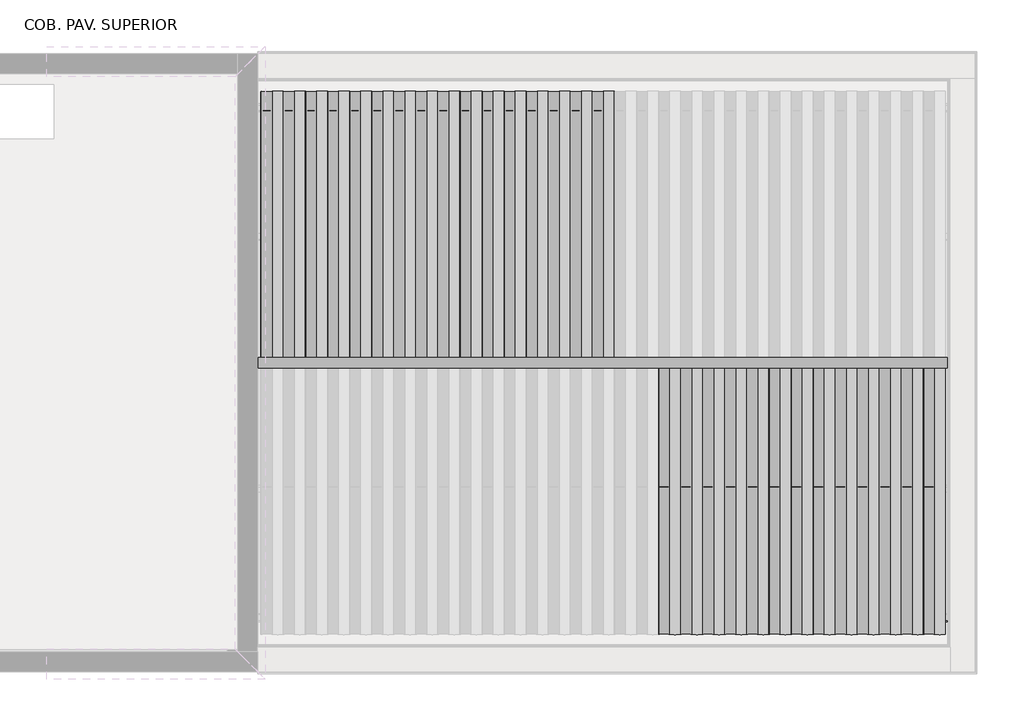
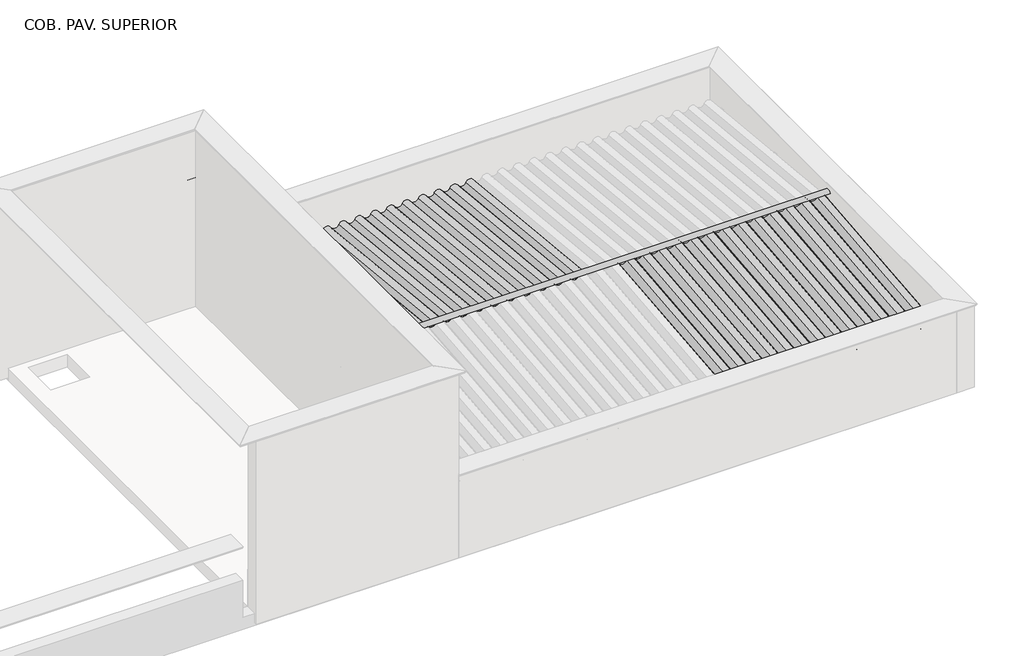
# One storey, part 6 of 7: 39 beams, 8 columns.
# Revit data of these elements (continued)
# Type "Madeira de lei : Berço 6x12cm"
#   A = 0.02 m²
#   Length [instance default] = 1.524 m
#   b = 0.06 m
#   d = 0.12 m
#   Structural Material [instance default] = none
#   Assembly Code = ""
# Type "Cumeeira Telha Ondulada : Fibrocimento"
#   Cost = 5
#   Length [instance default] = 1.524 m
#   b = 0.07 m
#   h = 0.16 m
#   Structural Material = .TELHA DE FIBROCIMENTO
#   Assembly Code = ""
# Type "Telha Ondulada : Fibrocimento"
#   Description = "TELHA ONDULADA FIBROCIMENTO"
#   Cost = 5
#   Length [instance default] = 1.524 m
#   b = 0.07 m
#   h = 0.16 m
#   Structural Material = .TELHA DE FIBROCIMENTO
#   Assembly Code = ""
# Type "Madeira de lei : Viga Cumeeira 6x16cm"
#   A = 0.02 m²
#   Length [instance default] = 1.524 m
#   b = 0.06 m
#   d = 0.16 m
#   Structural Material [instance default] = none
#   Assembly Code = ""
# Type "Madeira de lei-Coluna : Pontalete 6X16cm"
#   A = 0.01952 m²
#   b = 0.06 m
#   d = 0.16 m
#   Structural Material [instance default] = none
#   Assembly Code = ""
# Type "TQS - Pilar retangular : 19.0 x 30.0"
#   b = 0.19 m
#   h = 0.30 m
#   Structural Material [instance default] = Concrete - Cast-in-Place Concrete
# Elements 1, 2, 3, 4, 5, 6, 7, 8 (IfcBeam, "Madeira de lei : Berço 6x12cm")
#   Comments = ""
#   Structural Material = .MADEIRAMENTO
#   Phase Created = CC_PE
#   Materials on its faces: ".MADEIRAMENTO"
# Element 9 (IfcBeam, "Cumeeira Telha Ondulada : Fibrocimento")
#   Comments = ""
#   Phase Created = CC_PE
#   Materials on its faces: ".TELHA DE FIBROCIMENTO"
# Elements 10, 11, 12, 13, 14, 15, 16, 17, 18, 19, 20, 21, 22, 23, 24, 25, 26, 27, 28, 29, 30, 31, 32, 33, 34, 35, 36, 37, 38 (IfcBeam, "Telha Ondulada : Fibrocimento")
#   Phase Created = CC_PE
#   Materials on its faces: ".TELHA DE FIBROCIMENTO"
# Element 39 (IfcBeam, "Madeira de lei : Viga Cumeeira 6x16cm")
#   Comments = ""
#   Structural Material = .MADEIRAMENTO
#   Phase Created = CC_PE
#   Materials on its faces: ".MADEIRAMENTO"
# Elements 40, 41, 42, 43, 44, 45, 46 (IfcColumn, "Madeira de lei-Coluna : Pontalete 6X16cm")
#   Comments = ""
#   Structural Material = .MADEIRAMENTO
#   Phase Created = CC_PE
#   Materials on its faces: ".MADEIRAMENTO"
# Element 47 (IfcColumn, "TQS - Pilar retangular : 19.0 x 30.0")
#   Uso = "ESTRUTURA"
#   Titulo = "PT1"
#   Chave = "PT1//0"
#   Tipo Elemento = "Pilar"
#   SHA1 = "921092CA98E51B071105A8209417B462C0AB35B3"
#   Revisão = ""
#   Tipo de carga = ""
#   Divisor de flexao = ""
#   Secao = "R 19/30 90°"
#   Configuracao = ""
#   Angulo (graus) = ""
#   Detalhamento = ""
#   Casos de vento manual = ""
#   Tipo = ""
#   Alcas = ""
#   Furos = ""
#   Pino = ""
#   Distribuicao = ""
#   Solidarizado = ""
#   Solidarizar na montagem = ""
#   Unir com o próximo = ""
#   Grupo pre moldado = ""
#   Verificado = ""
#   Concreto C = ""
#   Taxa de armadura (kgf/m³) = 0
#   Carga (tf/m²) = 0
#   Carga (tf/m) = 0
#   Carga (tf) = 0
#   Altura = 2.10 m
#   Rebaixo = 0.00 m
#   Altura da fundacao = 0.00 m
#   Largura = 0.00 m
#   Distancia a face = 0.00 m
#   Distancia ao eixo = 0.00 m
#   Resultado de Ensaios fck (MPa) = 0
#   Unique TQS ID = -427
#   Principal = yes
#   Nasce = yes
#   Morre = yes
#   Cabeca de Pilar = no
#   Structural Material = Concrete - Cast-in-Place Concrete
#   Phase Created = CC_PE
#   Materials on its faces: "Concrete - Cast-in-Place Concrete"
# Materials
#   ".TELHA DE FIBROCIMENTO": class "CC_TELHADO", colour RGB 77 77 76, transparency 0, Description = "TELHA ONDULADA FIBROCIMENTO", Cost = 0
#   "Concrete - Cast-in-Place Concrete": class "Unassigned", colour RGB 192 192 192, transparency 0
#   ".MADEIRAMENTO": class ".CC_MADEIRAS", colour RGB 212 179 113, transparency 0, Cost = 0
